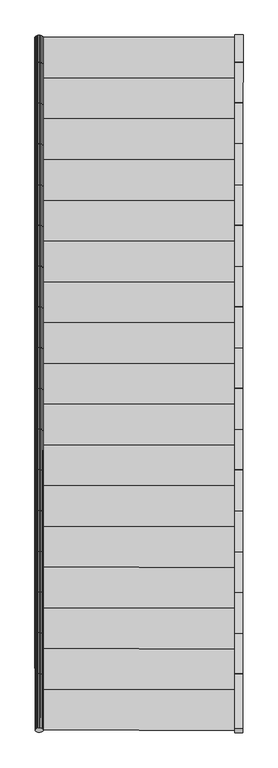
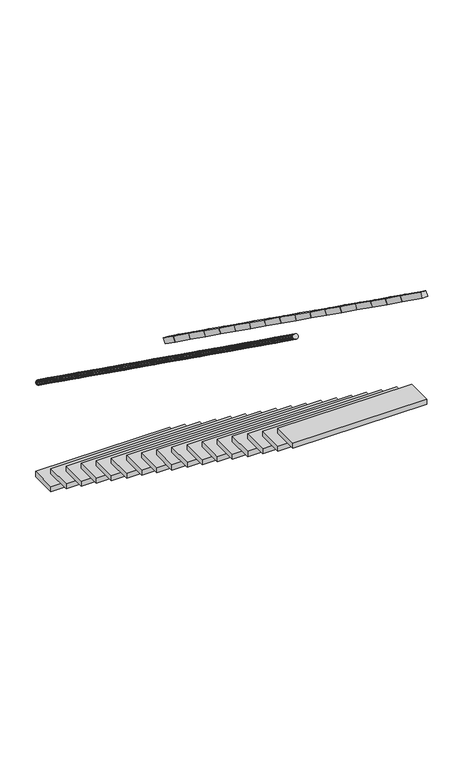
"""IFC4 building model written with IfcOpenShell, lengths in millimetres: stair geometry, 0_3d_modell."""

from ifc_helpers import new_model, si_unit, frame, origin, origin_with_axes, place, context, project, spatial, polyline, outline, extrude, faceted_brep, source, transform, mapped, element, save


def stair_cdc667ca(model_context):
    return source(origin(), model_context, "Body", "SolidModel", [
        extrude(outline(polyline([(1.2235871, -7.1914683), (0.0, 0.0), (1.2235871, 7.1914683), (4.7745752, 13.6789855), (10.3053687, 18.8275083), (17.2745752, 22.1330634), (25.0, 23.2720802), (32.7254248, 22.1330635), (39.6946313, 18.8275084), (45.2254249, 13.6789855), (48.7764129, 7.1914683), (50.0, 0.0), (48.7764129, -7.1914683), (45.2254249, -13.6789855), (39.6946313, -18.8275083), (32.7254249, -22.1330635), (25.0, -23.2720802), (17.2745751, -22.1330634), (10.3053687, -18.8275084), (4.7745751, -13.6789855), (1.2235871, -7.1914683)])), frame((0.0, 4178.4563133, 921.0), z_axis=(0.00011956441317344549, -0.8134084583000747, 0.5816929307377278), x_axis=(0.9999999891966984, 0.00014699184728057414, 0.0)), (0.0, 0.0, 1.0), 200.8460147),
        faceted_brep([(1.2841865, 3766.1927143, 1206.9811079), (0.0599845, 3770.3757605, 1212.8307092), (1.2829567, 3774.5591664, 1218.6803104), (4.83339, 3778.3334311, 1223.957312), (10.3637433, 3781.3291033, 1228.1451642), (17.332667, 3783.2529457, 1230.8339308), (25.0579944, 3783.9166392, 1231.7604166), (32.7835166, 3783.2552168, 1230.8339308), (39.7530056, 3781.3334233, 1228.1451642), (45.2842393, 3778.3393771, 1223.957312), (48.835782, 3774.5661563, 1218.6803104), (50.059984, 3770.3831101, 1212.8307092), (48.8370118, 3766.1997042, 1206.9811079), (45.2865785, 3762.4254395, 1201.7041063), (39.7562252, 3759.4297673, 1197.5162541), (32.7873015, 3757.5059249, 1194.8274876), (25.0619741, 3756.8422314, 1193.9010017), (17.3364519, 3757.5036538, 1194.8274876), (10.3669629, 3759.4254473, 1197.5162541), (4.8357292, 3762.4194935, 1201.7041063), (0.095955, 3525.6650407, 1387.8307114), (1.3189272, 3529.8484465, 1393.6803128), (4.8693605, 3533.622711, 1398.9573145), (10.3997137, 3536.6183831, 1403.1451667), (17.3686375, 3538.5422254, 1405.8339333), (25.0939649, 3539.2059189, 1406.7604192), (32.819487, 3538.5444966, 1405.8339333), (39.788976, 3536.6227031, 1403.1451667), (45.3202098, 3533.628657, 1398.9573145), (48.8717525, 3529.8554364, 1393.6803128), (50.0959545, 3525.6723903, 1387.8307114), (48.8729823, 3521.4889846, 1381.98111), (45.322549, 3517.71472, 1376.7041083), (39.7921957, 3514.719048, 1372.5162561), (32.823272, 3512.7952057, 1369.8274894), (25.0979446, 3512.1315122, 1368.9010036), (17.3724224, 3512.7929345, 1369.8274894), (10.4029334, 3514.714728, 1372.5162561), (4.8716997, 3517.7087741, 1376.7041083), (1.320157, 3521.4819947, 1381.98111)], [[[0, 1, 2, 3, 4, 5, 6, 7, 8, 9, 10, 11, 12, 13, 14, 15, 16, 17, 18, 19]], [[2, 1, 20, 21]], [[3, 2, 21, 22]], [[4, 3, 22, 23]], [[5, 4, 23, 24]], [[6, 5, 24, 25]], [[7, 6, 25, 26]], [[8, 7, 26, 27]], [[9, 8, 27, 28]], [[10, 9, 28, 29]], [[11, 10, 29, 30]], [[12, 11, 30, 31]], [[13, 12, 31, 32]], [[14, 13, 32, 33]], [[15, 14, 33, 34]], [[16, 15, 34, 35]], [[17, 16, 35, 36]], [[18, 17, 36, 37]], [[19, 18, 37, 38]], [[0, 19, 38, 39]], [[1, 0, 39, 20]], [[21, 20, 39, 38, 37, 36, 35, 34, 33, 32, 31, 30, 29, 28, 27, 26, 25, 24, 23, 22]]]),
        extrude(outline(polyline([(8.1923609, -49.3242862), (0.0, 0.0), (296.9699428, 49.3242863), (305.1623051, 2e-07), (8.1923609, -49.3242862)])), frame((1249.6184083, 1580.115245, 2807.2457343), z_axis=(-0.9999999892183941, 0.00014684417523468346, 0.0), x_axis=(-0.00013185515752107114, -0.8979256814680555, 0.4401470812970881)), (0.0, 0.0, 1.0), 50.0),
        extrude(outline(polyline([(1249.8920771, 3443.7838597), (1249.8561074, 3198.8318236), (0.143879, 3199.6331615), (0.1079093, 3444.3389707), (1249.8920771, 3443.7838597)])), frame((0.0, 0.0, 525.0), z_axis=(0.0, 0.0, 1.0), x_axis=(1.0, 0.0, 0.0)), (0.0, 0.0, 1.0), 50.0),
        faceted_brep([(1.320157, 3521.4819947, 1381.98111), (0.095955, 3525.6650407, 1387.8307114), (1.3189272, 3529.8484465, 1393.6803128), (4.8693605, 3533.6227111, 1398.9573145), (10.3997137, 3536.6183831, 1403.1451667), (17.3686375, 3538.5422254, 1405.8339333), (25.0939649, 3539.2059189, 1406.7604192), (32.819487, 3538.5444966, 1405.8339333), (39.788976, 3536.6227031, 1403.1451667), (45.3202098, 3533.628657, 1398.9573145), (48.8717525, 3529.8554364, 1393.6803128), (50.0959545, 3525.6723903, 1387.8307114), (48.8729823, 3521.4889846, 1381.98111), (45.322549, 3517.71472, 1376.7041083), (39.7921957, 3514.719048, 1372.5162561), (32.823272, 3512.7952057, 1369.8274894), (25.0979446, 3512.1315122, 1368.9010036), (17.3724224, 3512.7929345, 1369.8274894), (10.4029334, 3514.714728, 1372.5162561), (4.8716997, 3517.7087741, 1376.7041083), (0.1319255, 3280.9543068, 1562.8307136), (1.3548977, 3285.1377124, 1568.6803151), (4.905331, 3288.9119768, 1573.9573169), (10.4356842, 3291.9076488, 1578.1451692), (17.404608, 3293.831491, 1580.8339359), (25.1299354, 3294.4951844, 1581.7604218), (32.8554575, 3293.8337622, 1580.8339359), (39.8249465, 3291.9119688, 1578.1451692), (45.3561802, 3288.9179228, 1573.9573169), (48.907723, 3285.1447023, 1568.6803151), (50.1319249, 3280.9616564, 1562.8307136), (48.9089528, 3276.7782508, 1556.9811121), (45.3585195, 3273.0039864, 1551.7041103), (39.8281662, 3270.0083145, 1547.516258), (32.8592425, 3268.0844723, 1544.8274913), (25.1339151, 3267.4207788, 1543.9010054), (17.4083929, 3268.0822011, 1544.8274913), (10.4389039, 3270.0039945, 1547.516258), (4.9076702, 3272.9980405, 1551.7041103), (1.3561275, 3276.771261, 1556.9811121)], [[[0, 1, 2, 3, 4, 5, 6, 7, 8, 9, 10, 11, 12, 13, 14, 15, 16, 17, 18, 19]], [[2, 1, 20, 21]], [[3, 2, 21, 22]], [[4, 3, 22, 23]], [[5, 4, 23, 24]], [[6, 5, 24, 25]], [[7, 6, 25, 26]], [[8, 7, 26, 27]], [[9, 8, 27, 28]], [[10, 9, 28, 29]], [[11, 10, 29, 30]], [[12, 11, 30, 31]], [[13, 12, 31, 32]], [[14, 13, 32, 33]], [[15, 14, 33, 34]], [[16, 15, 34, 35]], [[17, 16, 35, 36]], [[18, 17, 36, 37]], [[19, 18, 37, 38]], [[0, 19, 38, 39]], [[1, 0, 39, 20]], [[21, 20, 39, 38, 37, 36, 35, 34, 33, 32, 31, 30, 29, 28, 27, 26, 25, 24, 23, 22]]]),
        extrude(outline(polyline([(8.1923597, -49.3242865), (0.0, 0.0), (296.9699893, 49.3242865), (305.1623504, 1e-07), (8.1923597, -49.3242865)])), frame((1249.7622844, 2559.9033777, 2107.2457448), z_axis=(-0.9999999892183942, 0.00014684417523692057, 0.0), x_axis=(-0.00013185516302004536, -0.8979257185584658, 0.44014700563048126)), (0.0, 0.0, 1.0), 50.0),
        extrude(outline(polyline([(8.1923591, -49.3242866), (0.0, 0.0), (296.9700126, 49.3242866), (305.162373, 2e-07), (8.1923591, -49.3242866)])), frame((1249.8342225, 3049.7975287, 1757.24575), z_axis=(-0.9999999892183942, 0.00014684417516961745, 0.0), x_axis=(-0.00013185516565950391, -0.8979257371398741, 0.44014696772331535)), (0.0, 0.0, 1.0), 50.0),
        extrude(outline(polyline([(8.19236, -49.3242866), (0.0, 0.0), (296.9699777, 49.3242864), (305.162339, 1e-07), (8.19236, -49.3242866)])), frame((1249.7263154, 2314.9563234, 2282.2457422), z_axis=(-0.9999999892183941, 0.00014684417524381637, 0.0), x_axis=(-0.00013185516158858616, -0.8979257092768325, 0.44014702456555777)), (0.0, 0.0, 1.0), 50.0),
        extrude(outline(polyline([(8.1923594, -49.3242866), (0.0, 0.0), (296.970001, 49.3242865), (305.1623617, 2e-07), (8.1923594, -49.3242866)])), frame((1249.7982535, 2804.8504462, 1932.2457474), z_axis=(-0.9999999892183941, 0.00014684417523698817, 0.0), x_axis=(-0.00013185516434937206, -0.8979257278461384, 0.44014698668308333)), (0.0, 0.0, 1.0), 50.0),
        extrude(outline(polyline([(1249.9999865, 4178.6400531), (1249.9640167, 3933.6879745), (0.0359698, 3933.7505466), (0.0, 4178.4563133), (1249.9999865, 4178.6400531)])), origin_with_axes(), (0.0, 0.0, 1.0), 50.0),
        extrude(outline(polyline([(8.1923585, -49.3242867), (0.0, 0.0), (296.9700359, 49.3242865), (305.1623957, 0.0), (8.1923585, -49.3242867)])), frame((1249.9061607, 3539.6917363, 1407.2457553), z_axis=(-0.9999999892183941, 0.00014684417518251225, 0.0), x_axis=(-0.0001318551683371763, -0.8979257557453363, 0.4401469297670736)), (0.0, 0.0, 1.0), 50.0),
        extrude(outline(polyline([(1249.9280469, 3688.73591), (1249.8920771, 3443.7838597), (0.1079093, 3444.3389707), (0.0719395, 3689.0447657), (1249.9280469, 3688.73591)])), frame((0.0, 0.0, 350.0), z_axis=(0.0, 0.0, 1.0), x_axis=(1.0, 0.0, 0.0)), (0.0, 0.0, 1.0), 50.0),
        faceted_brep([(1.248216, 4010.9034198, 1031.9811057), (0.024014, 4015.0864661, 1037.8307069), (1.2469862, 4019.2698722, 1043.6803081), (4.7974195, 4023.044137, 1048.9573096), (10.3277728, 4026.0398093, 1053.1451616), (17.2966965, 4027.9636518, 1055.8339282), (25.0220239, 4028.6273453, 1056.760414), (32.7475461, 4027.9659229, 1055.8339282), (39.7170351, 4026.0441293, 1053.1451616), (45.2482688, 4023.050083, 1048.9573096), (48.7998115, 4019.276862, 1043.6803081), (50.0240135, 4015.0938157, 1037.8307069), (48.8010413, 4010.9104096, 1031.9811057), (45.250608, 4007.1361448, 1026.7041043), (39.7202547, 4004.1404725, 1022.5162522), (32.751331, 4002.21663, 1019.8274857), (25.0260036, 4001.5529365, 1018.9009999), (17.3004815, 4002.2143589, 1019.8274857), (10.3309924, 4004.1361525, 1022.5162522), (4.7997587, 4007.1301988, 1026.7041043), (0.0599845, 3770.3757605, 1212.8307092), (1.2829567, 3774.5591664, 1218.6803104), (4.83339, 3778.3334311, 1223.957312), (10.3637433, 3781.3291033, 1228.1451642), (17.332667, 3783.2529457, 1230.8339308), (25.0579944, 3783.9166392, 1231.7604166), (32.7835166, 3783.2552168, 1230.8339308), (39.7530056, 3781.3334233, 1228.1451642), (45.2842393, 3778.3393771, 1223.957312), (48.835782, 3774.5661563, 1218.6803104), (50.059984, 3770.3831101, 1212.8307092), (48.8370118, 3766.1997042, 1206.9811079), (45.2865785, 3762.4254395, 1201.7041063), (39.7562252, 3759.4297673, 1197.5162541), (32.7873015, 3757.5059249, 1194.8274876), (25.0619741, 3756.8422314, 1193.9010017), (17.3364519, 3757.5036538, 1194.8274876), (10.3669629, 3759.4254473, 1197.5162541), (4.8357292, 3762.4194935, 1201.7041063), (1.2841865, 3766.1927143, 1206.9811079)], [[[0, 1, 2, 3, 4, 5, 6, 7, 8, 9, 10, 11, 12, 13, 14, 15, 16, 17, 18, 19]], [[2, 1, 20, 21]], [[3, 2, 21, 22]], [[4, 3, 22, 23]], [[5, 4, 23, 24]], [[6, 5, 24, 25]], [[7, 6, 25, 26]], [[8, 7, 26, 27]], [[9, 8, 27, 28]], [[10, 9, 28, 29]], [[11, 10, 29, 30]], [[12, 11, 30, 31]], [[13, 12, 31, 32]], [[14, 13, 32, 33]], [[15, 14, 33, 34]], [[16, 15, 34, 35]], [[17, 16, 35, 36]], [[18, 17, 36, 37]], [[19, 18, 37, 38]], [[0, 19, 38, 39]], [[1, 0, 39, 20]], [[21, 20, 39, 38, 37, 36, 35, 34, 33, 32, 31, 30, 29, 28, 27, 26, 25, 24, 23, 22]]]),
        extrude(outline(polyline([(1249.5323794, 994.2641337), (1249.4964097, 749.3122386), (0.5035767, 752.5742931), (0.467607, 997.2802433), (1249.5323794, 994.2641337)])), frame((0.0, 0.0, 2275.0), z_axis=(0.0, 0.0, 1.0), x_axis=(1.0, 0.0, 0.0)), (0.0, 0.0, 1.0), 50.0),
        faceted_brep([(1.6079209, 1563.7957291, 2781.9811268), (0.3837189, 1567.9787738, 2787.8307292), (1.6066911, 1572.1621783, 2793.6803315), (5.1571244, 1575.9364417, 2798.957334), (10.6874777, 1578.9321128, 2803.1451869), (17.6564014, 1580.8559545, 2805.8339539), (25.3817288, 1581.5196478, 2806.7604399), (33.107251, 1580.8582257, 2805.8339539), (40.07674, 1578.9364328, 2803.1451869), (45.6079737, 1575.9423876, 2798.957334), (49.1595164, 1572.1691682, 2793.6803315), (50.3837184, 1567.9861234, 2787.8307292), (49.1607462, 1563.8027189, 2781.9811268), (45.6103129, 1560.0284555, 2776.7041243), (40.0799596, 1557.0327844, 2772.5162715), (33.1110359, 1555.1089427, 2769.8275044), (25.3857085, 1554.4452494, 2768.9010184), (17.6601863, 1555.1066715, 2769.8275044), (10.6906973, 1557.0284644, 2772.5162715), (5.1594636, 1560.0225096, 2776.7041243), (0.4196894, 1323.267927, 2962.8307314), (1.6426616, 1327.4513313, 2968.6803338), (5.1930949, 1331.2255945, 2973.9573364), (10.7234482, 1334.2212656, 2978.1451894), (17.6923719, 1336.1451072, 2980.8339565), (25.4176993, 1336.8088004, 2981.7604425), (33.1432215, 1336.1473784, 2980.8339565), (40.1127105, 1334.2255855, 2978.1451894), (45.6439442, 1331.2315405, 2973.9573364), (49.1954869, 1327.4583212, 2968.6803338), (50.4196889, 1323.2752766, 2962.8307314), (49.1967167, 1319.0918723, 2956.9811289), (45.6462834, 1315.317609, 2951.7041263), (40.1159301, 1312.321938, 2947.5162734), (33.1470064, 1310.3980963, 2944.8275062), (25.421679, 1309.7344031, 2943.9010202), (17.6961568, 1310.3958252, 2944.8275062), (10.7266678, 1312.317618, 2947.5162734), (5.1954341, 1315.311663, 2951.7041263), (1.6438914, 1319.0848824, 2956.9811289)], [[[0, 1, 2, 3, 4, 5, 6, 7, 8, 9, 10, 11, 12, 13, 14, 15, 16, 17, 18, 19]], [[2, 1, 20, 21]], [[3, 2, 21, 22]], [[4, 3, 22, 23]], [[5, 4, 23, 24]], [[6, 5, 24, 25]], [[7, 6, 25, 26]], [[8, 7, 26, 27]], [[9, 8, 27, 28]], [[10, 9, 28, 29]], [[11, 10, 29, 30]], [[12, 11, 30, 31]], [[13, 12, 31, 32]], [[14, 13, 32, 33]], [[15, 14, 33, 34]], [[16, 15, 34, 35]], [[17, 16, 35, 36]], [[18, 17, 36, 37]], [[19, 18, 37, 38]], [[0, 19, 38, 39]], [[1, 0, 39, 20]], [[21, 20, 39, 38, 37, 36, 35, 34, 33, 32, 31, 30, 29, 28, 27, 26, 25, 24, 23, 22]]]),
        extrude(outline(polyline([(1249.8201376, 2953.8798016), (1249.7841678, 2708.9277937), (0.2158186, 2710.2215007), (0.1798488, 2954.9273381), (1249.8201376, 2953.8798016)])), frame((0.0, 0.0, 875.0), z_axis=(0.0, 0.0, 1.0), x_axis=(1.0, 0.0, 0.0)), (0.0, 0.0, 1.0), 50.0),
        faceted_brep([(1.7518029, 584.9522579, 3481.9811352), (0.5276009, 589.135302, 3487.830738), (1.7505731, 593.3187059, 3493.6803408), (5.3010064, 597.0929687, 3498.9573437), (10.8313597, 600.0886394, 3503.1451969), (17.8002834, 602.0124808, 3505.8339642), (25.5256108, 602.676174, 3506.7604502), (33.251133, 602.014752, 3505.8339642), (40.220622, 600.0929594, 3503.1451969), (45.7518557, 597.0989147, 3498.9573437), (49.3033984, 593.3256958, 3493.6803408), (50.5276004, 589.1426516, 3487.830738), (49.3046282, 584.9592478, 3481.9811352), (45.7541949, 581.184985, 3476.7041323), (40.2238416, 578.1893143, 3472.5162791), (33.2549179, 576.2654729, 3469.8275118), (25.5295905, 575.6017797, 3468.9010258), (17.8040684, 576.2632017, 3469.8275118), (10.8345793, 578.1849943, 3472.5162791), (5.3033456, 581.179039, 3476.7041323), (0.5635714, 344.424399, 3662.8307402), (1.7865436, 348.6078026, 3668.6803431), (5.3369769, 352.3820653, 3673.9573461), (10.8673302, 355.3777359, 3678.1451994), (17.8362539, 357.3015773, 3680.8339667), (25.5615813, 357.9652704, 3681.7604528), (33.2871035, 357.3038484, 3680.8339667), (40.2565925, 355.3820559, 3678.1451994), (45.7878262, 352.3880113, 3673.9573461), (49.3393689, 348.6147925, 3668.6803431), (50.5635709, 344.4317486, 3662.8307402), (49.3405987, 340.2483449, 3656.9811373), (45.7901654, 336.4740822, 3651.7041343), (40.2598121, 333.4784116, 3647.516281), (33.2908884, 331.5545703, 3644.8275137), (25.565561, 330.8908771, 3643.9010276), (17.8400389, 331.5522991, 3644.8275137), (10.8705499, 333.4740916, 3647.516281), (5.3393161, 336.4681363, 3651.7041343), (1.7877734, 340.241355, 3656.9811373)], [[[0, 1, 2, 3, 4, 5, 6, 7, 8, 9, 10, 11, 12, 13, 14, 15, 16, 17, 18, 19]], [[2, 1, 20, 21]], [[3, 2, 21, 22]], [[4, 3, 22, 23]], [[5, 4, 23, 24]], [[6, 5, 24, 25]], [[7, 6, 25, 26]], [[8, 7, 26, 27]], [[9, 8, 27, 28]], [[10, 9, 28, 29]], [[11, 10, 29, 30]], [[12, 11, 30, 31]], [[13, 12, 31, 32]], [[14, 13, 32, 33]], [[15, 14, 33, 34]], [[16, 15, 34, 35]], [[17, 16, 35, 36]], [[18, 17, 36, 37]], [[19, 18, 37, 38]], [[0, 19, 38, 39]], [[1, 0, 39, 20]], [[21, 20, 39, 38, 37, 36, 35, 34, 33, 32, 31, 30, 29, 28, 27, 26, 25, 24, 23, 22]]]),
        extrude(outline(polyline([(8.1923612, -49.3242862), (0.0, 0.0), (296.9699313, 49.3242862), (305.1622938, 1e-07), (8.1923612, -49.3242862)])), frame((1249.5824392, 1335.1682471, 2982.2457317), z_axis=(-0.9999999892183942, 0.0001468441751931061, 0.0), x_axis=(-0.0001318551561423782, -0.897925672210508, 0.4401471001830244)), (0.0, 0.0, 1.0), 50.0),
        extrude(outline(polyline([(8.1923603, -49.3242865), (0.0, 0.0), (296.9699661, 49.3242863), (305.1623277, 1e-07), (8.1923603, -49.3242865)])), frame((1249.6903463, 2070.0092832, 2457.2457396), z_axis=(-0.9999999892183942, 0.00014684417521627555, 0.0), x_axis=(-0.00013185516021942966, -0.897925700001208, 0.4401470434883751)), (0.0, 0.0, 1.0), 50.0),
        extrude(outline(polyline([(1249.7841678, 2708.9277937), (1249.748198, 2463.9758), (0.2517883, 2465.5156491), (0.2158186, 2710.2215007), (1249.7841678, 2708.9277937)])), frame((0.0, 0.0, 1050.0), z_axis=(0.0, 0.0, 1.0), x_axis=(1.0, 0.0, 0.0)), (0.0, 0.0, 1.0), 50.0),
        extrude(outline(polyline([(1249.4244702, 259.4084905), (1249.3885004, 14.4566375), (0.6114861, 18.4563582), (0.5755163, 263.1623506), (1249.4244702, 259.4084905)])), frame((0.0, 0.0, 2800.0), z_axis=(0.0, 0.0, 1.0), x_axis=(1.0, 0.0, 0.0)), (0.0, 0.0, 1.0), 50.0),
        faceted_brep([(1.4280684, 2787.349751, 1906.9811163), (0.2038665, 2791.5327966, 1912.8307181), (1.4268386, 2795.7162018, 1918.6803198), (4.9772719, 2799.490466, 1923.9573218), (10.5076252, 2802.4861377, 1928.1451743), (17.4765489, 2804.4099798, 1930.8339411), (25.2018763, 2805.0736731, 1931.760427), (32.9273985, 2804.4122509, 1930.8339411), (39.8968875, 2802.4904577, 1928.1451743), (45.4281212, 2799.4964119, 1923.9573218), (48.9796639, 2795.7231917, 1918.6803198), (50.2038659, 2791.5401462, 1912.8307181), (48.9808937, 2787.3567409, 1906.9811163), (45.4304604, 2783.5824768, 1901.7041143), (39.9001072, 2780.5868051, 1897.5162619), (32.9311834, 2778.662963, 1894.827495), (25.205856, 2777.9992696, 1893.9010091), (17.4803339, 2778.6606918, 1894.827495), (10.5108449, 2780.5824851, 1897.5162619), (4.9796112, 2783.5765308, 1901.7041143), (0.2398369, 2546.8220202, 2087.8307203), (1.4628091, 2551.0054253, 2093.6803221), (5.0132424, 2554.7796893, 2098.9573242), (10.5435957, 2557.7753609, 2103.1451768), (17.5125194, 2559.6992029, 2105.8339436), (25.2378468, 2560.3628963, 2106.7604296), (32.963369, 2559.7014741, 2105.8339436), (39.932858, 2557.7796809, 2103.1451768), (45.4640917, 2554.7856353, 2098.9573242), (49.0156344, 2551.0124152, 2093.6803221), (50.2398364, 2546.8293698, 2087.8307203), (49.0168642, 2542.6459647, 2081.9811184), (45.4664309, 2538.8717007, 2076.7041163), (39.9360776, 2535.8760291, 2072.5162638), (32.9671539, 2533.9521871, 2069.8274969), (25.2418265, 2533.2884938, 2068.901011), (17.5163044, 2533.949916, 2069.8274969), (10.5468154, 2535.8717092, 2072.5162638), (5.0155816, 2538.8657548, 2076.7041163), (1.4640389, 2542.6389748, 2081.9811184)], [[[0, 1, 2, 3, 4, 5, 6, 7, 8, 9, 10, 11, 12, 13, 14, 15, 16, 17, 18, 19]], [[2, 1, 20, 21]], [[3, 2, 21, 22]], [[4, 3, 22, 23]], [[5, 4, 23, 24]], [[6, 5, 24, 25]], [[7, 6, 25, 26]], [[8, 7, 26, 27]], [[9, 8, 27, 28]], [[10, 9, 28, 29]], [[11, 10, 29, 30]], [[12, 11, 30, 31]], [[13, 12, 31, 32]], [[14, 13, 32, 33]], [[15, 14, 33, 34]], [[16, 15, 34, 35]], [[17, 16, 35, 36]], [[18, 17, 36, 37]], [[19, 18, 37, 38]], [[0, 19, 38, 39]], [[1, 0, 39, 20]], [[21, 20, 39, 38, 37, 36, 35, 34, 33, 32, 31, 30, 29, 28, 27, 26, 25, 24, 23, 22]]]),
        faceted_brep([(1.7877734, 340.241355, 3656.9811373), (0.5635714, 344.424399, 3662.8307402), (1.7865436, 348.6078026, 3668.6803431), (5.3369769, 352.3820653, 3673.9573461), (10.8673302, 355.3777359, 3678.1451994), (17.8362539, 357.3015773, 3680.8339667), (25.5615813, 357.9652704, 3681.7604528), (33.2871035, 357.3038484, 3680.8339667), (40.2565925, 355.3820559, 3678.1451994), (45.7878262, 352.3880113, 3673.9573461), (49.3393689, 348.6147925, 3668.6803431), (50.5635709, 344.4317486, 3662.8307402), (49.3405987, 340.2483449, 3656.9811373), (45.7901654, 336.4740822, 3651.7041343), (40.2598121, 333.4784116, 3647.516281), (33.2908884, 331.5545703, 3644.8275137), (25.565561, 330.8908771, 3643.9010276), (17.8400389, 331.5522991, 3644.8275137), (10.8705499, 333.4740916, 3647.516281), (5.3393161, 336.4681363, 3651.7041343), (0.6114984, 18.3726106, 3896.0), (1.8344706, 22.5560142, 3901.849603), (5.3849039, 26.3302767, 3907.1266061), (10.9152571, 29.3259472, 3911.3144595), (17.8841809, 31.2497884, 3914.0032269), (25.6095083, 31.9134815, 3914.929713), (33.3350304, 31.2520596, 3914.0032269), (40.3045194, 29.3302671, 3911.3144595), (45.8357532, 26.3362226, 3907.1266061), (49.3872959, 22.563004, 3901.849603), (50.6114979, 18.3799602, 3896.0), (49.3885257, 14.1965567, 3890.150397), (45.8380924, 10.4222942, 3884.8733939), (40.3077391, 7.4266237, 3880.6855405), (33.3388154, 5.5027824, 3877.9967731), (25.613488, 4.8390893, 3877.070287), (17.8879658, 5.5005113, 3877.9967731), (10.9184768, 7.4223037, 3880.6855405), (5.3872431, 10.4163482, 3884.8733939), (1.8357004, 14.1895668, 3890.150397)], [[[0, 1, 2, 3, 4, 5, 6, 7, 8, 9, 10, 11, 12, 13, 14, 15, 16, 17, 18, 19]], [[2, 1, 20, 21]], [[3, 2, 21, 22]], [[4, 3, 22, 23]], [[5, 4, 23, 24]], [[6, 5, 24, 25]], [[7, 6, 25, 26]], [[8, 7, 26, 27]], [[9, 8, 27, 28]], [[10, 9, 28, 29]], [[11, 10, 29, 30]], [[12, 11, 30, 31]], [[13, 12, 31, 32]], [[14, 13, 32, 33]], [[15, 14, 33, 34]], [[16, 15, 34, 35]], [[17, 16, 35, 36]], [[18, 17, 36, 37]], [[19, 18, 37, 38]], [[0, 19, 38, 39]], [[1, 0, 39, 20]], [[21, 20, 39, 38, 37, 36, 35, 34, 33, 32, 31, 30, 29, 28, 27, 26, 25, 24, 23, 22]]]),
        extrude(outline(polyline([(12.0678028, -48.5218315), (0.0, 0.0), (195.0950121, 48.5218316), (207.1628149, 0.0), (12.0678028, -48.5218315)])), frame((1249.9978513, 4164.0996769, 899.6941742), z_axis=(8.536363471883801e-05, 0.5813212113037808, 0.8136741620583482), x_axis=(-0.24147200455189077, -0.7895837620479879, 0.5641354037177938)), (0.0, 0.0, 1.0), 50.0),
        extrude(outline(polyline([(1249.748198, 2463.9758), (1249.7122283, 2219.0238204), (0.2877581, 2220.8097833), (0.2517883, 2465.5156491), (1249.748198, 2463.9758)])), frame((0.0, 0.0, 1225.0), z_axis=(0.0, 0.0, 1.0), x_axis=(1.0, 0.0, 0.0)), (0.0, 0.0, 1.0), 50.0),
        extrude(outline(polyline([(8.1923615, -49.3242863), (0.0, 0.0), (296.9699197, 49.3242861), (305.1622825, 1e-07), (8.1923615, -49.3242863)])), frame((1249.5464702, 1090.2212632, 3157.2457291), z_axis=(-0.9999999892183941, 0.00014684417527455952, 0.0), x_axis=(-0.00013185515474304962, -0.8979256629590162, 0.44014711905660536)), (0.0, 0.0, 1.0), 50.0),
        faceted_brep([(1.3561275, 3276.771261, 1556.9811121), (0.1319255, 3280.9543068, 1562.8307136), (1.3548977, 3285.1377124, 1568.6803151), (4.905331, 3288.9119768, 1573.9573169), (10.4356842, 3291.9076488, 1578.1451692), (17.404608, 3293.831491, 1580.8339359), (25.1299354, 3294.4951844, 1581.7604218), (32.8554575, 3293.8337622, 1580.8339359), (39.8249465, 3291.9119688, 1578.1451692), (45.3561802, 3288.9179228, 1573.9573169), (48.907723, 3285.1447023, 1568.6803151), (50.1319249, 3280.9616564, 1562.8307136), (48.9089528, 3276.7782508, 1556.9811121), (45.3585195, 3273.0039864, 1551.7041103), (39.8281662, 3270.0083145, 1547.516258), (32.8592425, 3268.0844723, 1544.8274913), (25.1339151, 3267.4207788, 1543.9010054), (17.4083929, 3268.0822011, 1544.8274913), (10.4389039, 3270.0039945, 1547.516258), (4.9076702, 3272.9980405, 1551.7041103), (0.167896, 3036.2435588, 1737.8307158), (1.3908681, 3040.4269642, 1743.6803175), (4.9413014, 3044.2012285, 1748.9573193), (10.4716547, 3047.1969003, 1753.1451717), (17.4405785, 3049.1207424, 1755.8339385), (25.1659058, 3049.7844359, 1756.7604244), (32.891428, 3049.1230136, 1755.8339385), (39.860917, 3047.2012203, 1753.1451717), (45.3921507, 3044.2071744, 1748.9573193), (48.9436934, 3040.4339541, 1743.6803175), (50.1678954, 3036.2509084, 1737.8307158), (48.9449232, 3032.0675029, 1731.9811142), (45.3944899, 3028.2932387, 1726.7041123), (39.8641367, 3025.2975668, 1722.5162599), (32.8952129, 3023.3737247, 1719.8274932), (25.1698856, 3022.7100313, 1718.9010073), (17.4443634, 3023.3714535, 1719.8274932), (10.4748744, 3025.2932469, 1722.5162599), (4.9436407, 3028.2872927, 1726.7041123), (1.3920979, 3032.0605131, 1731.9811142)], [[[0, 1, 2, 3, 4, 5, 6, 7, 8, 9, 10, 11, 12, 13, 14, 15, 16, 17, 18, 19]], [[2, 1, 20, 21]], [[3, 2, 21, 22]], [[4, 3, 22, 23]], [[5, 4, 23, 24]], [[6, 5, 24, 25]], [[7, 6, 25, 26]], [[8, 7, 26, 27]], [[9, 8, 27, 28]], [[10, 9, 28, 29]], [[11, 10, 29, 30]], [[12, 11, 30, 31]], [[13, 12, 31, 32]], [[14, 13, 32, 33]], [[15, 14, 33, 34]], [[16, 15, 34, 35]], [[17, 16, 35, 36]], [[18, 17, 36, 37]], [[19, 18, 37, 38]], [[0, 19, 38, 39]], [[1, 0, 39, 20]], [[21, 20, 39, 38, 37, 36, 35, 34, 33, 32, 31, 30, 29, 28, 27, 26, 25, 24, 23, 22]]]),
        extrude(outline(polyline([(1249.604319, 1484.1679662), (1249.5683492, 1239.2160429), (0.4316372, 1241.9861795), (0.3956674, 1486.6921016), (1249.604319, 1484.1679662)])), frame((0.0, 0.0, 1925.0), z_axis=(0.0, 0.0, 1.0), x_axis=(1.0, 0.0, 0.0)), (0.0, 0.0, 1.0), 50.0),
        extrude(outline(polyline([(1249.9640167, 3933.6879745), (1249.9280469, 3688.73591), (0.0719395, 3689.0447657), (0.0359698, 3933.7505466), (1249.9640167, 3933.6879745)])), frame((0.0, 0.0, 175.0), z_axis=(0.0, 0.0, 1.0), x_axis=(1.0, 0.0, 0.0)), (0.0, 0.0, 1.0), 50.0),
        extrude(outline(polyline([(8.1923588, -49.3242867), (0.0, 0.0), (296.9700243, 49.3242866), (305.1623844, 2e-07), (8.1923588, -49.3242867)])), frame((1249.8701916, 3294.7446254, 1582.2457526), z_axis=(-0.9999999892183942, 0.0001468441753055469, 0.0), x_axis=(-0.00013185516714837089, -0.8979257464395866, 0.4401469487513531)), (0.0, 0.0, 1.0), 50.0),
        faceted_brep([(1.7158324, 829.6631468, 3306.9811331), (0.4916304, 833.8461911, 3312.8307358), (1.7146026, 838.0295951, 3318.6803385), (5.2650359, 841.803858, 3323.9573413), (10.7953892, 844.7995288, 3328.1451944), (17.7643129, 846.7233703, 3330.8339616), (25.4896403, 847.3870635, 3331.7604477), (33.2151625, 846.7256415, 3330.8339616), (40.1846515, 844.8038488, 3328.1451944), (45.7158852, 841.809804, 3323.9573413), (49.2674279, 838.0365849, 3318.6803385), (50.4916299, 833.8535407, 3312.8307358), (49.2686577, 829.6701367, 3306.9811331), (45.7182244, 825.8958737, 3301.7041303), (40.1878711, 822.9002029, 3297.5162772), (33.2189474, 820.9763614, 3294.82751), (25.49362, 820.3126682, 3293.9010239), (17.7680978, 820.9740903, 3294.82751), (10.7986088, 822.8958829, 3297.5162772), (5.2673751, 825.8899278, 3301.7041303), (0.5276009, 589.135302, 3487.830738), (1.7505731, 593.3187059, 3493.6803408), (5.3010064, 597.0929687, 3498.9573437), (10.8313597, 600.0886394, 3503.1451969), (17.8002834, 602.0124808, 3505.8339642), (25.5256108, 602.676174, 3506.7604502), (33.251133, 602.014752, 3505.8339642), (40.220622, 600.0929594, 3503.1451969), (45.7518557, 597.0989147, 3498.9573437), (49.3033984, 593.3256958, 3493.6803408), (50.5276004, 589.1426516, 3487.830738), (49.3046282, 584.9592478, 3481.9811352), (45.7541949, 581.184985, 3476.7041323), (40.2238416, 578.1893143, 3472.5162791), (33.2549179, 576.2654729, 3469.8275118), (25.5295905, 575.6017797, 3468.9010258), (17.8040684, 576.2632017, 3469.8275118), (10.8345793, 578.1849943, 3472.5162791), (5.3033456, 581.179039, 3476.7041323), (1.7518029, 584.9522579, 3481.9811352)], [[[0, 1, 2, 3, 4, 5, 6, 7, 8, 9, 10, 11, 12, 13, 14, 15, 16, 17, 18, 19]], [[2, 1, 20, 21]], [[3, 2, 21, 22]], [[4, 3, 22, 23]], [[5, 4, 23, 24]], [[6, 5, 24, 25]], [[7, 6, 25, 26]], [[8, 7, 26, 27]], [[9, 8, 27, 28]], [[10, 9, 28, 29]], [[11, 10, 29, 30]], [[12, 11, 30, 31]], [[13, 12, 31, 32]], [[14, 13, 32, 33]], [[15, 14, 33, 34]], [[16, 15, 34, 35]], [[17, 16, 35, 36]], [[18, 17, 36, 37]], [[19, 18, 37, 38]], [[0, 19, 38, 39]], [[1, 0, 39, 20]], [[21, 20, 39, 38, 37, 36, 35, 34, 33, 32, 31, 30, 29, 28, 27, 26, 25, 24, 23, 22]]]),
        extrude(outline(polyline([(1249.4964097, 749.3122386), (1249.4604399, 504.3603576), (0.5395465, 507.8683289), (0.5035767, 752.5742931), (1249.4964097, 749.3122386)])), frame((0.0, 0.0, 2450.0), z_axis=(0.0, 0.0, 1.0), x_axis=(1.0, 0.0, 0.0)), (0.0, 0.0, 1.0), 50.0),
        extrude(outline(polyline([(1249.8561074, 3198.8318236), (1249.8201376, 2953.8798016), (0.1798488, 2954.9273381), (0.143879, 3199.6331615), (1249.8561074, 3198.8318236)])), frame((0.0, 0.0, 700.0), z_axis=(0.0, 0.0, 1.0), x_axis=(1.0, 0.0, 0.0)), (0.0, 0.0, 1.0), 50.0),
        extrude(outline(polyline([(8.1923582, -49.3242868), (0.0, 0.0), (296.9700476, 49.3242867), (305.1624071, 1e-07), (8.1923582, -49.3242868)])), frame((1249.9421297, 3784.6388613, 1232.2457579), z_axis=(-0.9999999892183942, 0.00014684417521348882, 0.0), x_axis=(-0.0001318551698676997, -0.8979257650571499, 0.44014691077042245)), (0.0, 0.0, 1.0), 50.0),
        extrude(outline(polyline([(8.1923618, -49.3242862), (0.0, 0.0), (296.9699081, 49.3242861), (305.1622712, 1e-07), (8.1923618, -49.3242862)])), frame((1249.5105011, 845.2742934, 3332.2457265), z_axis=(-0.9999999892183942, 0.00014684417542298043, 0.0), x_axis=(-0.00013185515363887585, -0.8979256537135019, 0.44014713791799076)), (0.0, 0.0, 1.0), 50.0),
        extrude(outline(polyline([(8.1923606, -49.3242864), (0.0, 0.0), (296.9699545, 49.3242862), (305.1623164, 1e-07), (8.1923606, -49.3242864)])), frame((1249.6543773, 1825.0622571, 2632.245737), z_axis=(-0.9999999892183942, 0.00014684417531856612, 0.0), x_axis=(-0.00013185515896060372, -0.8979256907316218, 0.44014706239887275)), (0.0, 0.0, 1.0), 50.0),
        faceted_brep([(1.5000094, 2297.9281846, 2256.9811205), (0.2758074, 2302.1112298, 2262.8307225), (1.4987796, 2306.2946347, 2268.6803245), (5.0492129, 2310.0688986, 2273.9573267), (10.5795662, 2313.0645701, 2278.1451793), (17.5484899, 2314.988412, 2280.8339462), (25.2738173, 2315.6521053, 2281.7604322), (32.9993395, 2314.9906831, 2280.8339462), (39.9688285, 2313.06889, 2278.1451793), (45.5000622, 2310.0748445, 2273.9573267), (49.0516049, 2306.3016246, 2268.6803245), (50.2758069, 2302.1185794, 2262.8307225), (49.0528347, 2297.9351744, 2256.9811205), (45.5024014, 2294.1609106, 2251.7041183), (39.9720481, 2291.1652391, 2247.5162657), (33.0031244, 2289.2413972, 2244.8274988), (25.277797, 2288.5777038, 2243.9010128), (17.5522749, 2289.239126, 2244.8274988), (10.5827858, 2291.1609191, 2247.5162657), (5.0515521, 2294.1549647, 2251.7041183), (0.3117779, 2057.4004252, 2437.8307247), (1.5347501, 2061.58383, 2443.6803268), (5.0851834, 2065.3580937, 2448.9573291), (10.6155367, 2068.3537651, 2453.1451818), (17.5844604, 2070.2776069, 2455.8339488), (25.3097878, 2070.9413003, 2456.7604347), (33.03531, 2070.2798781, 2455.8339488), (40.004799, 2068.3580851, 2453.1451818), (45.5360327, 2065.3640396, 2448.9573291), (49.0875754, 2061.5908199, 2443.6803268), (50.3117774, 2057.4077748, 2437.8307247), (49.0888052, 2053.22437, 2431.9811226), (45.5383719, 2049.4501063, 2426.7041203), (40.0080186, 2046.454435, 2422.5162676), (33.0390949, 2044.5305931, 2419.8275007), (25.3137675, 2043.8668998, 2418.9010147), (17.5882453, 2044.528322, 2419.8275007), (10.6187563, 2046.450115, 2422.5162676), (5.0875226, 2049.4441604, 2426.7041203), (1.5359799, 2053.2173802, 2431.9811226)], [[[0, 1, 2, 3, 4, 5, 6, 7, 8, 9, 10, 11, 12, 13, 14, 15, 16, 17, 18, 19]], [[2, 1, 20, 21]], [[3, 2, 21, 22]], [[4, 3, 22, 23]], [[5, 4, 23, 24]], [[6, 5, 24, 25]], [[7, 6, 25, 26]], [[8, 7, 26, 27]], [[9, 8, 27, 28]], [[10, 9, 28, 29]], [[11, 10, 29, 30]], [[12, 11, 30, 31]], [[13, 12, 31, 32]], [[14, 13, 32, 33]], [[15, 14, 33, 34]], [[16, 15, 34, 35]], [[17, 16, 35, 36]], [[18, 17, 36, 37]], [[19, 18, 37, 38]], [[0, 19, 38, 39]], [[1, 0, 39, 20]], [[21, 20, 39, 38, 37, 36, 35, 34, 33, 32, 31, 30, 29, 28, 27, 26, 25, 24, 23, 22]]]),
        faceted_brep([(1.4640389, 2542.6389748, 2081.9811184), (0.2398369, 2546.8220202, 2087.8307203), (1.4628091, 2551.0054253, 2093.6803221), (5.0132424, 2554.7796893, 2098.9573242), (10.5435957, 2557.7753609, 2103.1451768), (17.5125194, 2559.6992029, 2105.8339436), (25.2378468, 2560.3628963, 2106.7604296), (32.963369, 2559.7014741, 2105.8339436), (39.932858, 2557.7796809, 2103.1451768), (45.4640917, 2554.7856353, 2098.9573242), (49.0156344, 2551.0124152, 2093.6803221), (50.2398364, 2546.8293698, 2087.8307203), (49.0168642, 2542.6459647, 2081.9811184), (45.4664309, 2538.8717007, 2076.7041163), (39.9360776, 2535.8760291, 2072.5162638), (32.9671539, 2533.9521871, 2069.8274969), (25.2418265, 2533.2884938, 2068.901011), (17.5163044, 2533.949916, 2069.8274969), (10.5468154, 2535.8717092, 2072.5162638), (5.0155816, 2538.8657548, 2076.7041163), (0.2758074, 2302.1112298, 2262.8307225), (1.4987796, 2306.2946347, 2268.6803245), (5.0492129, 2310.0688986, 2273.9573267), (10.5795662, 2313.0645701, 2278.1451793), (17.5484899, 2314.988412, 2280.8339462), (25.2738173, 2315.6521053, 2281.7604322), (32.9993395, 2314.9906831, 2280.8339462), (39.9688285, 2313.06889, 2278.1451793), (45.5000622, 2310.0748445, 2273.9573267), (49.0516049, 2306.3016246, 2268.6803245), (50.2758069, 2302.1185794, 2262.8307225), (49.0528347, 2297.9351744, 2256.9811205), (45.5024014, 2294.1609106, 2251.7041183), (39.9720481, 2291.1652391, 2247.5162657), (33.0031244, 2289.2413972, 2244.8274988), (25.277797, 2288.5777038, 2243.9010128), (17.5522749, 2289.239126, 2244.8274988), (10.5827858, 2291.1609191, 2247.5162657), (5.0515521, 2294.1549647, 2251.7041183), (1.5000094, 2297.9281846, 2256.9811205)], [[[0, 1, 2, 3, 4, 5, 6, 7, 8, 9, 10, 11, 12, 13, 14, 15, 16, 17, 18, 19]], [[2, 1, 20, 21]], [[3, 2, 21, 22]], [[4, 3, 22, 23]], [[5, 4, 23, 24]], [[6, 5, 24, 25]], [[7, 6, 25, 26]], [[8, 7, 26, 27]], [[9, 8, 27, 28]], [[10, 9, 28, 29]], [[11, 10, 29, 30]], [[12, 11, 30, 31]], [[13, 12, 31, 32]], [[14, 13, 32, 33]], [[15, 14, 33, 34]], [[16, 15, 34, 35]], [[17, 16, 35, 36]], [[18, 17, 36, 37]], [[19, 18, 37, 38]], [[0, 19, 38, 39]], [[1, 0, 39, 20]], [[21, 20, 39, 38, 37, 36, 35, 34, 33, 32, 31, 30, 29, 28, 27, 26, 25, 24, 23, 22]]]),
        extrude(outline(polyline([(1249.4604399, 504.3603576), (1249.4244702, 259.4084905), (0.5755163, 263.1623506), (0.5395465, 507.8683289), (1249.4604399, 504.3603576)])), frame((0.0, 0.0, 2625.0), z_axis=(0.0, 0.0, 1.0), x_axis=(1.0, 0.0, 0.0)), (0.0, 0.0, 1.0), 50.0),
        faceted_brep([(1.6438914, 1319.0848824, 2956.9811289), (0.4196894, 1323.267927, 2962.8307314), (1.6426616, 1327.4513313, 2968.6803338), (5.1930949, 1331.2255945, 2973.9573364), (10.7234482, 1334.2212656, 2978.1451894), (17.6923719, 1336.1451072, 2980.8339565), (25.4176993, 1336.8088004, 2981.7604425), (33.1432215, 1336.1473784, 2980.8339565), (40.1127105, 1334.2255855, 2978.1451894), (45.6439442, 1331.2315405, 2973.9573364), (49.1954869, 1327.4583212, 2968.6803338), (50.4196889, 1323.2752766, 2962.8307314), (49.1967167, 1319.0918723, 2956.9811289), (45.6462834, 1315.317609, 2951.7041263), (40.1159301, 1312.321938, 2947.5162734), (33.1470064, 1310.3980963, 2944.8275062), (25.421679, 1309.7344031, 2943.9010202), (17.6961568, 1310.3958252, 2944.8275062), (10.7266678, 1312.317618, 2947.5162734), (5.1954341, 1315.311663, 2951.7041263), (0.4556599, 1078.5570661, 3137.8307336), (1.6786321, 1082.7404702, 3143.6803361), (5.2290654, 1086.5147333, 3148.9573388), (10.7594187, 1089.5104042, 3153.1451919), (17.7283424, 1091.4342458, 3155.833959), (25.4536698, 1092.097939, 3156.7604451), (33.179192, 1091.436517, 3155.833959), (40.148681, 1089.5147242, 3153.1451919), (45.6799147, 1086.5206793, 3148.9573388), (49.2314574, 1082.7474601, 3143.6803361), (50.4556594, 1078.5644156, 3137.8307336), (49.2326872, 1074.3810115, 3131.981131), (45.6822539, 1070.6067484, 3126.7041283), (40.1519006, 1067.6110775, 3122.5162753), (33.1829769, 1065.6872359, 3119.8275081), (25.4576495, 1065.0235427, 3118.9010221), (17.7321273, 1065.6849647, 3119.8275081), (10.7626383, 1067.6067575, 3122.5162753), (5.2314046, 1070.6008024, 3126.7041283), (1.6798619, 1074.3740216, 3131.981131)], [[[0, 1, 2, 3, 4, 5, 6, 7, 8, 9, 10, 11, 12, 13, 14, 15, 16, 17, 18, 19]], [[2, 1, 20, 21]], [[3, 2, 21, 22]], [[4, 3, 22, 23]], [[5, 4, 23, 24]], [[6, 5, 24, 25]], [[7, 6, 25, 26]], [[8, 7, 26, 27]], [[9, 8, 27, 28]], [[10, 9, 28, 29]], [[11, 10, 29, 30]], [[12, 11, 30, 31]], [[13, 12, 31, 32]], [[14, 13, 32, 33]], [[15, 14, 33, 34]], [[16, 15, 34, 35]], [[17, 16, 35, 36]], [[18, 17, 36, 37]], [[19, 18, 37, 38]], [[0, 19, 38, 39]], [[1, 0, 39, 20]], [[21, 20, 39, 38, 37, 36, 35, 34, 33, 32, 31, 30, 29, 28, 27, 26, 25, 24, 23, 22]]]),
        extrude(outline(polyline([(6.1859269, -49.6158675), (0.0, 0.0), (397.9571628, 49.6158674), (404.143091, 1e-07), (6.1859269, -49.6158675)])), frame((1249.4385631, 355.380396, 3682.2457213), z_axis=(-0.9999999892183942, 0.0001468441750629601, 0.0), x_axis=(-0.00012912639818669227, -0.8793429948958728, 0.47618891277929865)), (0.0, 0.0, 1.0), 50.0),
        faceted_brep([(1.6798619, 1074.3740216, 3131.981131), (0.4556599, 1078.5570661, 3137.8307336), (1.6786321, 1082.7404702, 3143.6803361), (5.2290654, 1086.5147333, 3148.9573388), (10.7594187, 1089.5104042, 3153.1451919), (17.7283424, 1091.4342458, 3155.833959), (25.4536698, 1092.097939, 3156.7604451), (33.179192, 1091.436517, 3155.833959), (40.148681, 1089.5147242, 3153.1451919), (45.6799147, 1086.5206793, 3148.9573388), (49.2314574, 1082.7474601, 3143.6803361), (50.4556594, 1078.5644156, 3137.8307336), (49.2326872, 1074.3810115, 3131.981131), (45.6822539, 1070.6067484, 3126.7041283), (40.1519006, 1067.6110775, 3122.5162753), (33.1829769, 1065.6872359, 3119.8275081), (25.4576495, 1065.0235427, 3118.9010221), (17.7321273, 1065.6849647, 3119.8275081), (10.7626383, 1067.6067575, 3122.5162753), (5.2314046, 1070.6008024, 3126.7041283), (0.4916304, 833.8461911, 3312.8307358), (1.7146026, 838.0295951, 3318.6803385), (5.2650359, 841.803858, 3323.9573413), (10.7953892, 844.7995288, 3328.1451944), (17.7643129, 846.7233703, 3330.8339616), (25.4896403, 847.3870635, 3331.7604477), (33.2151625, 846.7256415, 3330.8339616), (40.1846515, 844.8038488, 3328.1451944), (45.7158852, 841.809804, 3323.9573413), (49.2674279, 838.0365849, 3318.6803385), (50.4916299, 833.8535407, 3312.8307358), (49.2686577, 829.6701367, 3306.9811331), (45.7182244, 825.8958737, 3301.7041303), (40.1878711, 822.9002029, 3297.5162772), (33.2189474, 820.9763614, 3294.82751), (25.49362, 820.3126682, 3293.9010239), (17.7680978, 820.9740903, 3294.82751), (10.7986088, 822.8958829, 3297.5162772), (5.2673751, 825.8899278, 3301.7041303), (1.7158324, 829.6631468, 3306.9811331)], [[[0, 1, 2, 3, 4, 5, 6, 7, 8, 9, 10, 11, 12, 13, 14, 15, 16, 17, 18, 19]], [[2, 1, 20, 21]], [[3, 2, 21, 22]], [[4, 3, 22, 23]], [[5, 4, 23, 24]], [[6, 5, 24, 25]], [[7, 6, 25, 26]], [[8, 7, 26, 27]], [[9, 8, 27, 28]], [[10, 9, 28, 29]], [[11, 10, 29, 30]], [[12, 11, 30, 31]], [[13, 12, 31, 32]], [[14, 13, 32, 33]], [[15, 14, 33, 34]], [[16, 15, 34, 35]], [[17, 16, 35, 36]], [[18, 17, 36, 37]], [[19, 18, 37, 38]], [[0, 19, 38, 39]], [[1, 0, 39, 20]], [[21, 20, 39, 38, 37, 36, 35, 34, 33, 32, 31, 30, 29, 28, 27, 26, 25, 24, 23, 22]]]),
        faceted_brep([(1.5359799, 2053.2173802, 2431.9811226), (0.3117779, 2057.4004252, 2437.8307247), (1.5347501, 2061.58383, 2443.6803268), (5.0851834, 2065.3580937, 2448.9573291), (10.6155367, 2068.3537651, 2453.1451818), (17.5844604, 2070.2776069, 2455.8339488), (25.3097878, 2070.9413003, 2456.7604347), (33.03531, 2070.2798781, 2455.8339488), (40.004799, 2068.3580851, 2453.1451818), (45.5360327, 2065.3640396, 2448.9573291), (49.0875754, 2061.5908199, 2443.6803268), (50.3117774, 2057.4077748, 2437.8307247), (49.0888052, 2053.22437, 2431.9811226), (45.5383719, 2049.4501063, 2426.7041203), (40.0080186, 2046.454435, 2422.5162676), (33.0390949, 2044.5305931, 2419.8275007), (25.3137675, 2043.8668998, 2418.9010147), (17.5882453, 2044.528322, 2419.8275007), (10.6187563, 2046.450115, 2422.5162676), (5.0875226, 2049.4441604, 2426.7041203), (0.3477484, 1812.6896066, 2612.8307269), (1.5707206, 1816.8730112, 2618.6803291), (5.1211539, 1820.6472747, 2623.9573315), (10.6515072, 1823.642946, 2628.1451843), (17.6204309, 1825.5667878, 2630.8339514), (25.3457583, 1826.2304811, 2631.7604373), (33.0712805, 1825.5690589, 2630.8339514), (40.0407695, 1823.647266, 2628.1451843), (45.5720032, 1820.6532207, 2623.9573315), (49.1235459, 1816.8800011, 2618.6803291), (50.3477479, 1812.6969562, 2612.8307269), (49.1247757, 1808.5135515, 2606.9811247), (45.5743424, 1804.739288, 2601.7041223), (40.0439891, 1801.7436167, 2597.5162695), (33.0750654, 1799.8197749, 2594.8275025), (25.349738, 1799.1560816, 2593.9010165), (17.6242158, 1799.8175038, 2594.8275025), (10.6547268, 1801.7392967, 2597.5162695), (5.1234931, 1804.733342, 2601.7041223), (1.5719504, 1808.5065616, 2606.9811247)], [[[0, 1, 2, 3, 4, 5, 6, 7, 8, 9, 10, 11, 12, 13, 14, 15, 16, 17, 18, 19]], [[2, 1, 20, 21]], [[3, 2, 21, 22]], [[4, 3, 22, 23]], [[5, 4, 23, 24]], [[6, 5, 24, 25]], [[7, 6, 25, 26]], [[8, 7, 26, 27]], [[9, 8, 27, 28]], [[10, 9, 28, 29]], [[11, 10, 29, 30]], [[12, 11, 30, 31]], [[13, 12, 31, 32]], [[14, 13, 32, 33]], [[15, 14, 33, 34]], [[16, 15, 34, 35]], [[17, 16, 35, 36]], [[18, 17, 36, 37]], [[19, 18, 37, 38]], [[0, 19, 38, 39]], [[1, 0, 39, 20]], [[21, 20, 39, 38, 37, 36, 35, 34, 33, 32, 31, 30, 29, 28, 27, 26, 25, 24, 23, 22]]]),
        faceted_brep([(1.3920979, 3032.0605131, 1731.9811142), (0.167896, 3036.2435588, 1737.8307158), (1.3908681, 3040.4269642, 1743.6803175), (4.9413014, 3044.2012285, 1748.9573193), (10.4716547, 3047.1969003, 1753.1451717), (17.4405785, 3049.1207424, 1755.8339385), (25.1659058, 3049.7844359, 1756.7604244), (32.891428, 3049.1230136, 1755.8339385), (39.860917, 3047.2012203, 1753.1451717), (45.3921507, 3044.2071744, 1748.9573193), (48.9436934, 3040.4339541, 1743.6803175), (50.1678954, 3036.2509084, 1737.8307158), (48.9449232, 3032.0675029, 1731.9811142), (45.3944899, 3028.2932387, 1726.7041123), (39.8641367, 3025.2975668, 1722.5162599), (32.8952129, 3023.3737247, 1719.8274932), (25.1698856, 3022.7100313, 1718.9010073), (17.4443634, 3023.3714535, 1719.8274932), (10.4748744, 3025.2932469, 1722.5162599), (4.9436407, 3028.2872927, 1726.7041123), (0.2038665, 2791.5327966, 1912.8307181), (1.4268386, 2795.7162018, 1918.6803198), (4.9772719, 2799.490466, 1923.9573218), (10.5076252, 2802.4861377, 1928.1451743), (17.4765489, 2804.4099798, 1930.8339411), (25.2018763, 2805.0736731, 1931.760427), (32.9273985, 2804.4122509, 1930.8339411), (39.8968875, 2802.4904577, 1928.1451743), (45.4281212, 2799.4964119, 1923.9573218), (48.9796639, 2795.7231917, 1918.6803198), (50.2038659, 2791.5401462, 1912.8307181), (48.9808937, 2787.3567409, 1906.9811163), (45.4304604, 2783.5824768, 1901.7041143), (39.9001072, 2780.5868051, 1897.5162619), (32.9311834, 2778.662963, 1894.827495), (25.205856, 2777.9992696, 1893.9010091), (17.4803339, 2778.6606918, 1894.827495), (10.5108449, 2780.5824851, 1897.5162619), (4.9796112, 2783.5765308, 1901.7041143), (1.4280684, 2787.349751, 1906.9811163)], [[[0, 1, 2, 3, 4, 5, 6, 7, 8, 9, 10, 11, 12, 13, 14, 15, 16, 17, 18, 19]], [[2, 1, 20, 21]], [[3, 2, 21, 22]], [[4, 3, 22, 23]], [[5, 4, 23, 24]], [[6, 5, 24, 25]], [[7, 6, 25, 26]], [[8, 7, 26, 27]], [[9, 8, 27, 28]], [[10, 9, 28, 29]], [[11, 10, 29, 30]], [[12, 11, 30, 31]], [[13, 12, 31, 32]], [[14, 13, 32, 33]], [[15, 14, 33, 34]], [[16, 15, 34, 35]], [[17, 16, 35, 36]], [[18, 17, 36, 37]], [[19, 18, 37, 38]], [[0, 19, 38, 39]], [[1, 0, 39, 20]], [[21, 20, 39, 38, 37, 36, 35, 34, 33, 32, 31, 30, 29, 28, 27, 26, 25, 24, 23, 22]]]),
        extrude(outline(polyline([(1249.6402887, 1729.1199035), (1249.604319, 1484.1679662), (0.3956674, 1486.6921016), (0.3596976, 1731.3980096), (1249.6402887, 1729.1199035)])), frame((0.0, 0.0, 1750.0), z_axis=(0.0, 0.0, 1.0), x_axis=(1.0, 0.0, 0.0)), (0.0, 0.0, 1.0), 50.0),
        extrude(outline(polyline([(1249.6762585, 1974.0718549), (1249.6402887, 1729.1199035), (0.3596976, 1731.3980096), (0.3237279, 1976.1039035), (1249.6762585, 1974.0718549)])), frame((0.0, 0.0, 1575.0), z_axis=(0.0, 0.0, 1.0), x_axis=(1.0, 0.0, 0.0)), (0.0, 0.0, 1.0), 50.0),
        extrude(outline(polyline([(1249.7122283, 2219.0238204), (1249.6762585, 1974.0718549), (0.3237279, 1976.1039035), (0.2877581, 2220.8097833), (1249.7122283, 2219.0238204)])), frame((0.0, 0.0, 1400.0), z_axis=(0.0, 0.0, 1.0), x_axis=(1.0, 0.0, 0.0)), (0.0, 0.0, 1.0), 50.0),
        faceted_brep([(1.5719504, 1808.5065616, 2606.9811247), (0.3477484, 1812.6896066, 2612.8307269), (1.5707206, 1816.8730112, 2618.6803291), (5.1211539, 1820.6472747, 2623.9573315), (10.6515072, 1823.642946, 2628.1451843), (17.6204309, 1825.5667878, 2630.8339514), (25.3457583, 1826.2304811, 2631.7604373), (33.0712805, 1825.5690589, 2630.8339514), (40.0407695, 1823.647266, 2628.1451843), (45.5720032, 1820.6532207, 2623.9573315), (49.1235459, 1816.8800011, 2618.6803291), (50.3477479, 1812.6969562, 2612.8307269), (49.1247757, 1808.5135515, 2606.9811247), (45.5743424, 1804.739288, 2601.7041223), (40.0439891, 1801.7436167, 2597.5162695), (33.0750654, 1799.8197749, 2594.8275025), (25.349738, 1799.1560816, 2593.9010165), (17.6242158, 1799.8175038, 2594.8275025), (10.6547268, 1801.7392967, 2597.5162695), (5.1234931, 1804.733342, 2601.7041223), (0.3837189, 1567.9787738, 2787.8307292), (1.6066911, 1572.1621783, 2793.6803315), (5.1571244, 1575.9364417, 2798.957334), (10.6874777, 1578.9321128, 2803.1451869), (17.6564014, 1580.8559545, 2805.8339539), (25.3817288, 1581.5196478, 2806.7604399), (33.107251, 1580.8582257, 2805.8339539), (40.07674, 1578.9364328, 2803.1451869), (45.6079737, 1575.9423876, 2798.957334), (49.1595164, 1572.1691682, 2793.6803315), (50.3837184, 1567.9861234, 2787.8307292), (49.1607462, 1563.8027189, 2781.9811268), (45.6103129, 1560.0284555, 2776.7041243), (40.0799596, 1557.0327844, 2772.5162715), (33.1110359, 1555.1089427, 2769.8275044), (25.3857085, 1554.4452494, 2768.9010184), (17.6601863, 1555.1066715, 2769.8275044), (10.6906973, 1557.0284644, 2772.5162715), (5.1594636, 1560.0225096, 2776.7041243), (1.6079209, 1563.7957291, 2781.9811268)], [[[0, 1, 2, 3, 4, 5, 6, 7, 8, 9, 10, 11, 12, 13, 14, 15, 16, 17, 18, 19]], [[2, 1, 20, 21]], [[3, 2, 21, 22]], [[4, 3, 22, 23]], [[5, 4, 23, 24]], [[6, 5, 24, 25]], [[7, 6, 25, 26]], [[8, 7, 26, 27]], [[9, 8, 27, 28]], [[10, 9, 28, 29]], [[11, 10, 29, 30]], [[12, 11, 30, 31]], [[13, 12, 31, 32]], [[14, 13, 32, 33]], [[15, 14, 33, 34]], [[16, 15, 34, 35]], [[17, 16, 35, 36]], [[18, 17, 36, 37]], [[19, 18, 37, 38]], [[0, 19, 38, 39]], [[1, 0, 39, 20]], [[21, 20, 39, 38, 37, 36, 35, 34, 33, 32, 31, 30, 29, 28, 27, 26, 25, 24, 23, 22]]]),
        extrude(outline(polyline([(8.1923579, -49.3242869), (0.0, 0.0), (296.9700593, 49.3242867), (305.1624185, 1e-07), (8.1923579, -49.3242869)])), frame((1249.9780988, 4029.5860005, 1057.2457605), z_axis=(-0.9999999892183941, 0.00014684417520172762, 0.0), x_axis=(-0.00013185517118111294, -0.8979257743749991, 0.44014689176145727)), (0.0, 0.0, 1.0), 50.0),
        extrude(outline(polyline([(1249.5683492, 1239.2160429), (1249.5323794, 994.2641337), (0.467607, 997.2802433), (0.4316372, 1241.9861795), (1249.5683492, 1239.2160429)])), frame((0.0, 0.0, 2100.0), z_axis=(0.0, 0.0, 1.0), x_axis=(1.0, 0.0, 0.0)), (0.0, 0.0, 1.0), 50.0),
        extrude(outline(polyline([(8.1923621, -49.3242861), (0.0, 0.0), (296.9698965, 49.324286), (305.16226, 1e-07), (8.1923621, -49.3242861)])), frame((1249.4745321, 600.3273377, 3507.2457239), z_axis=(-0.9999999892183942, 0.00014684417504093425, 0.0), x_axis=(-0.00013185515200472844, -0.8979256444740168, 0.44014715676707555)), (0.0, 0.0, 1.0), 50.0),
    ])


if __name__ == "__main__":
    model = new_model("IFC4")
    model_context = context("Model", 3, world=origin())
    ifc_project = project(units=[si_unit("LENGTHUNIT", "METRE", prefix="MILLI")], contexts=[model_context])
    site = spatial("IfcSite", under=ifc_project)
    building = spatial("IfcBuilding", under=site)
    placement = place(None, origin())
    stair_shape = stair_cdc667ca(model_context)
    element("IfcStair", 1, ObjectType="0_3d_modell", at=placement, inside=building, context=model_context, shape_type="MappedRepresentation", body=[
        mapped(stair_shape, transform((0.0, 0.0, 0.0), x_axis=(1.0, 0.0, 0.0), y_axis=(0.0, 1.0, 0.0), z_axis=(0.0, 0.0, 1.0))),
    ])
    save(model, "model.ifc")

# Revit data of these elements
# Element 1 (IfcStair, "0_3d_modell")
#   Materials on its faces: "*1", "weiss"
# Materials
#   "*1": class "Unassigned", colour RGB 175 175 175, transparency 0
#   "weiss": class "Unassigned", colour RGB 255 255 255, transparency 0
